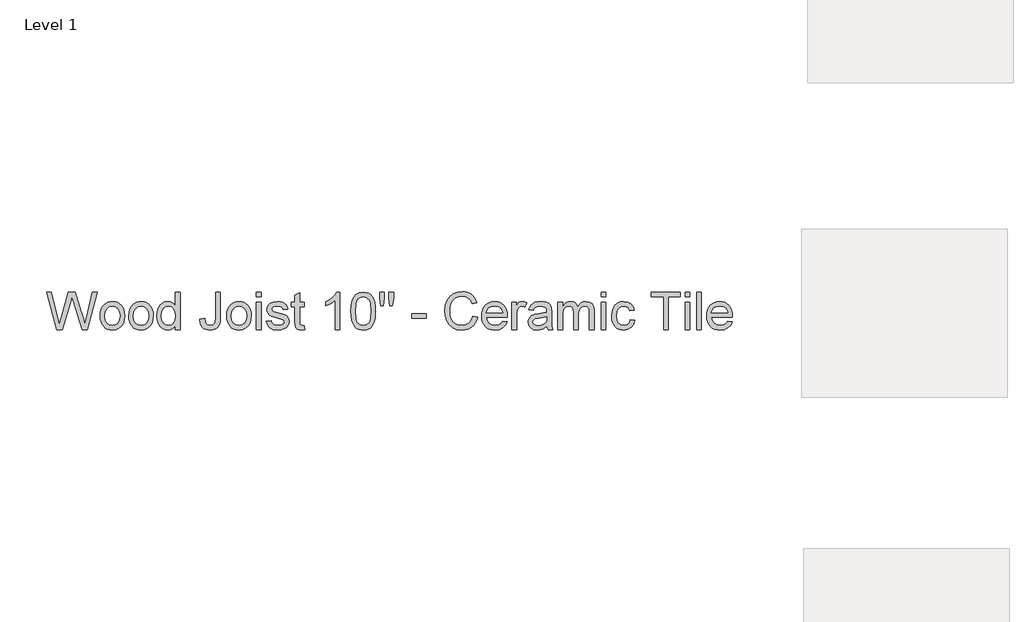
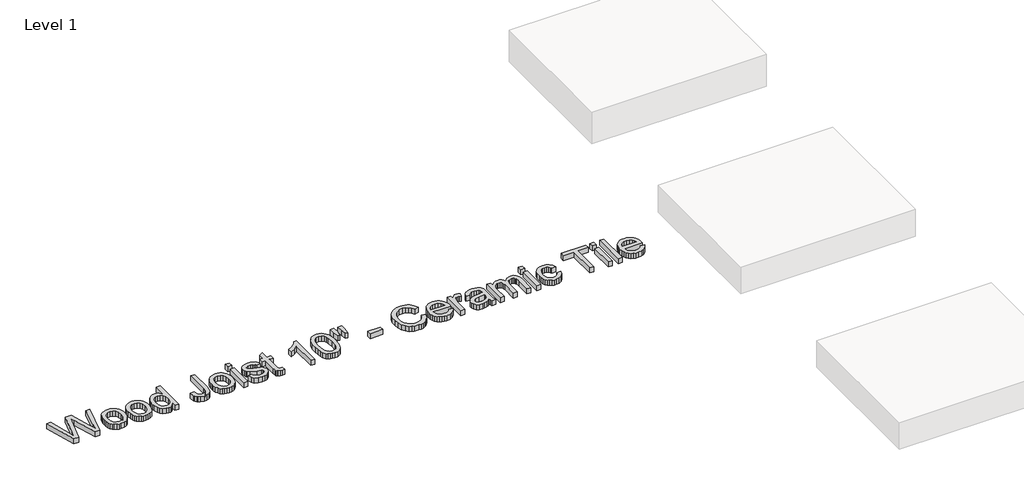
# One storey, part 15 of 42: 1 proxy.
"""IFC4 building model written with IfcOpenShell, lengths in millimetres."""

from ifc_helpers import new_model, si_unit, origin, origin_with_axes, place, context, project, spatial, polyline, outline, extrude, element, save

model = new_model("IFC4")

# Units and contexts
model_context = context("Model", 3, world=origin())
ifc_project = project(units=[si_unit("LENGTHUNIT", "METRE", prefix="MILLI")], contexts=[model_context])

# Site, building, storey
site = spatial("IfcSite", under=ifc_project)
building = spatial("IfcBuilding", under=site)
storey = spatial("IfcBuildingStorey", under=building, Name="Level 1", Elevation=0.0)

# Proxy
placement = place(None, origin())
element("IfcBuildingElementProxy", 1, Name="8\" Arial", ObjectType="8\" Arial", at=placement, inside=storey, context=model_context, shape_type="SweptSolid", body=[
    extrude(outline(polyline([(28459.9813839, -11347.8808193), (28376.9243908, -11043.3137252), (28416.1849927, -11043.3137252), (28464.3684588, -11243.4833095), (28479.2398989, -11305.2741433), (28495.1523399, -11250.6216008), (28555.5303868, -11043.3137252), (28612.1162166, -11043.3137252), (28655.986965, -11193.5896278), (28674.7807475, -11249.3575284), (28688.6297761, -11305.2741433), (28703.055073, -11245.2678823), (28751.6846823, -11043.3137252), (28790.9452843, -11043.3137252), (28707.8139339, -11347.8808193), (28667.1405451, -11347.8808193), (28594.121774, -11112.9120651), (28583.9348375, -11080.1205396), (28572.4838286, -11119.6042131), (28505.934134, -11347.8808193), (28459.9813839, -11347.8808193)])), origin_with_axes(), (0.0, 0.0, 1.0), 50.8),
    extrude(outline(polyline([(28814.7395885, -11236.0475894), (28816.7983535, -11207.0808124), (28822.9746485, -11182.1200296), (28833.2684734, -11161.165241), (28847.6798284, -11144.2164466), (28862.1887772, -11133.3835319), (28878.2034593, -11125.6457357), (28895.7238747, -11121.003058), (28914.7500234, -11119.4554987), (28935.753609, -11121.339989), (28954.7449027, -11126.99346), (28971.7239048, -11136.4159115), (28986.6906151, -11149.6073436), (28998.906109, -11166.1216132), (29007.6314617, -11185.5125769), (29012.8666734, -11207.7802349), (29014.611744, -11232.924587), (29011.5259201, -11271.3858491), (29002.2684486, -11300.6639968), (28987.1088743, -11322.5900764), (28966.3167421, -11338.9951338), (28941.6208568, -11349.2285435), (28914.7500234, -11352.6396801), (28893.4397144, -11350.7621608), (28874.2718223, -11345.1296029), (28857.246347, -11335.7420063), (28842.3632885, -11322.599371), (28830.2779198, -11305.9247688), (28821.6455135, -11285.9412711), (28816.4660697, -11262.648878), (28814.7395885, -11236.0475894)]), holes=[polyline([(28852.8104752, -11235.9732322), (28857.2161394, -11270.4285001), (28870.4331318, -11294.975671), (28890.323683, -11309.6705128), (28914.7500234, -11314.5687934), (28939.064828, -11309.6426288), (28958.9182006, -11294.8641352), (28972.1351931, -11269.9916516), (28976.5408572, -11234.783517), (28972.1073091, -11201.3320714), (28958.8066648, -11177.1195079), (28938.9254083, -11162.4246661), (28914.7500234, -11157.5263855), (28890.323683, -11162.4060768), (28870.4331318, -11177.0451507), (28857.2161394, -11201.5365537), (28852.8104752, -11235.9732322)])]), origin_with_axes(), (0.0, 0.0, 1.0), 50.8),
    extrude(outline(polyline([(29047.9237699, -11236.0475894), (29049.9825349, -11207.0808124), (29056.1588299, -11182.1200296), (29066.4526548, -11161.165241), (29080.8640098, -11144.2164466), (29095.3729586, -11133.3835319), (29111.3876407, -11125.6457357), (29128.9080561, -11121.003058), (29147.9342048, -11119.4554987), (29168.9377903, -11121.339989), (29187.9290841, -11126.99346), (29204.9080862, -11136.4159115), (29219.8747965, -11149.6073436), (29232.0902904, -11166.1216132), (29240.8156431, -11185.5125769), (29246.0508548, -11207.7802349), (29247.7959254, -11232.924587), (29244.7101015, -11271.3858491), (29235.45263, -11300.6639968), (29220.2930557, -11322.5900764), (29199.5009235, -11338.9951338), (29174.8050382, -11349.2285435), (29147.9342048, -11352.6396801), (29126.6238958, -11350.7621608), (29107.4560037, -11345.1296029), (29090.4305284, -11335.7420063), (29075.5474699, -11322.599371), (29063.4621012, -11305.9247688), (29054.8296949, -11285.9412711), (29049.6502511, -11262.648878), (29047.9237699, -11236.0475894)]), holes=[polyline([(29085.9946566, -11235.9732322), (29090.4003208, -11270.4285001), (29103.6173132, -11294.975671), (29123.5078644, -11309.6705128), (29147.9342048, -11314.5687934), (29172.2490094, -11309.6426288), (29192.102382, -11294.8641352), (29205.3193745, -11269.9916516), (29209.7250386, -11234.783517), (29205.2914905, -11201.3320714), (29191.9908462, -11177.1195079), (29172.1095897, -11162.4246661), (29147.9342048, -11157.5263855), (29123.5078644, -11162.4060768), (29103.6173132, -11177.0451507), (29090.4003208, -11201.5365537), (29085.9946566, -11235.9732322)])]), origin_with_axes(), (0.0, 0.0, 1.0), 50.8),
    extrude(outline(polyline([(29428.6326375, -11347.8808193), (29428.6326375, -11311.9662913), (29417.2420438, -11329.7608989), (29403.4441357, -11342.4713329), (29387.2389133, -11350.0975933), (29368.6263765, -11352.6396801), (29344.0141431, -11348.9589987), (29321.4839112, -11337.9169544), (29302.4112893, -11320.2850032), (29288.1718853, -11296.834601), (29279.3047892, -11268.5138022), (29276.3490904, -11236.270661), (29279.0724229, -11204.4271898), (29287.2424203, -11175.6695425), (29300.8497881, -11151.6335773), (29319.8852314, -11133.9551529), (29342.9080797, -11123.0804123), (29368.4776621, -11119.4554987), (29387.1041409, -11122.0487061), (29403.5742608, -11129.8283282), (29417.5348253, -11141.7533643), (29428.6326375, -11156.7828135), (29428.6326375, -11043.3137252), (29466.7035242, -11043.3137252), (29466.7035242, -11347.8808193), (29428.6326375, -11347.8808193)]), holes=[polyline([(29314.4199772, -11236.1219466), (29318.7141055, -11270.5586252), (29331.5964905, -11295.0500282), (29350.3159158, -11309.6891021), (29372.1211649, -11314.5687934), (29393.9171194, -11309.9121737), (29412.1625175, -11295.9423146), (29424.5151075, -11272.3989659), (29428.6326375, -11239.0218775), (29424.4407503, -11202.5310812), (29411.8650887, -11177.2310437), (29393.1549581, -11162.45255), (29370.5596637, -11157.5263855), (29348.531343, -11162.2573624), (29330.4811325, -11176.4502931), (29318.435266, -11200.8301603), (29314.4199772, -11236.1219466)])]), origin_with_axes(), (0.0, 0.0, 1.0), 50.8),
    extrude(outline(polyline([(29628.5047929, -11262.3700385), (29666.5756797, -11257.4624632), (29670.5352006, -11285.1419312), (29679.5881898, -11302.4485697), (29693.4186292, -11311.5387374), (29711.7105005, -11314.5687934), (29725.7733061, -11312.8492831), (29737.7726994, -11307.6907523), (29747.0301709, -11299.5672281), (29752.8672111, -11288.9527377), (29756.9940358, -11251.2164584), (29756.9940358, -11043.3137252), (29795.0649225, -11043.3137252), (29795.0649225, -11250.5472436), (29792.7691439, -11284.4448324), (29785.8818082, -11309.6983967), (29774.0032454, -11328.1482772), (29756.7337855, -11341.6348144), (29735.0493669, -11349.8884637), (29709.9259277, -11352.6396801), (29674.7363825, -11346.9606489), (29660.6410456, -11339.8618599), (29648.8786659, -11329.9235553), (29639.658373, -11317.1829137), (29633.1892966, -11301.6771137), (29628.5047929, -11262.3700385)])), origin_with_axes(), (0.0, 0.0, 1.0), 50.8),
    extrude(outline(polyline([(29847.4123918, -11236.0475894), (29849.4711568, -11207.0808124), (29855.6474518, -11182.1200296), (29865.9412768, -11161.165241), (29880.3526317, -11144.2164466), (29894.8615805, -11133.3835319), (29910.8762626, -11125.6457357), (29928.396678, -11121.003058), (29947.4228267, -11119.4554987), (29968.4264123, -11121.339989), (29987.4177061, -11126.99346), (30004.3967081, -11136.4159115), (30019.3634184, -11149.6073436), (30031.5789123, -11166.1216132), (30040.3042651, -11185.5125769), (30045.5394767, -11207.7802349), (30047.2845473, -11232.924587), (30044.1987235, -11271.3858491), (30034.941252, -11300.6639968), (30019.7816777, -11322.5900764), (29998.9895454, -11338.9951338), (29974.2936601, -11349.2285435), (29947.4228267, -11352.6396801), (29926.1125178, -11350.7621608), (29906.9446256, -11345.1296029), (29889.9191503, -11335.7420063), (29875.0360919, -11322.599371), (29862.9507231, -11305.9247688), (29854.3183168, -11285.9412711), (29849.1388731, -11262.648878), (29847.4123918, -11236.0475894)]), holes=[polyline([(29885.4832786, -11235.9732322), (29889.8889427, -11270.4285001), (29903.1059351, -11294.975671), (29922.9964863, -11309.6705128), (29947.4228267, -11314.5687934), (29971.7376314, -11309.6426288), (29991.591004, -11294.8641352), (30004.8079964, -11269.9916516), (30009.2136605, -11234.783517), (30004.7801124, -11201.3320714), (29991.4794682, -11177.1195079), (29971.5982116, -11162.4246661), (29947.4228267, -11157.5263855), (29922.9964863, -11162.4060768), (29903.1059351, -11177.0451507), (29889.8889427, -11201.5365537), (29885.4832786, -11235.9732322)])]), origin_with_axes(), (0.0, 0.0, 1.0), 50.8),
    extrude(outline(polyline([(30090.1142949, -11347.8808193), (30090.1142949, -11124.2143596), (30128.1851816, -11124.2143596), (30128.1851816, -11347.8808193), (30090.1142949, -11347.8808193)])), origin_with_axes(), (0.0, 0.0, 1.0), 50.8),
    extrude(outline(polyline([(30090.1142949, -11081.384612), (30090.1142949, -11043.3137252), (30128.1851816, -11043.3137252), (30128.1851816, -11081.384612), (30090.1142949, -11081.384612)])), origin_with_axes(), (0.0, 0.0, 1.0), 50.8),
    extrude(outline(polyline([(30171.0149292, -11281.2567675), (30209.085816, -11276.4979066), (30215.09016, -11292.7821336), (30226.7084726, -11304.7536429), (30244.015111, -11312.1150057), (30267.0844326, -11314.5687934), (30289.8749146, -11312.3194881), (30305.8988913, -11305.5715721), (30315.3794344, -11295.7936002), (30318.5396154, -11284.4541271), (30315.3608451, -11274.7505124), (30305.8245341, -11267.3519709), (30266.6382893, -11256.4958196), (30209.3088876, -11237.8693409), (30194.7999388, -11228.5096282), (30184.2876896, -11216.1198596), (30177.902265, -11201.4900804), (30175.7737901, -11185.4103358), (30177.4840057, -11170.6597261), (30182.6146526, -11157.0430637), (30190.7009981, -11145.0994383), (30201.2783099, -11135.3679397), (30225.4815788, -11124.1028238), (30258.2359257, -11119.4554987), (30283.0154628, -11121.3237234), (30304.5604617, -11126.9283974), (30321.8856895, -11135.7211364), (30334.0059132, -11147.153556), (30342.0364909, -11162.0714694), (30347.0927805, -11181.3206897), (30309.0218937, -11186.0795506), (30304.2165597, -11174.0987466), (30294.7081326, -11165.0736414), (30280.4036661, -11159.4131995), (30261.2102137, -11157.5263855), (30239.3491967, -11159.3295476), (30224.7751854, -11164.739034), (30216.577304, -11172.54654), (30213.8446769, -11181.5437613), (30218.3804661, -11192.6229842), (30232.5826914, -11201.0253479), (30265.3742169, -11209.1302828), (30321.2536533, -11227.0503681), (30336.0135576, -11235.6200355), (30347.2043163, -11247.3498839), (30354.2589557, -11262.277092), (30356.6105022, -11280.4388383), (30353.8499911, -11299.2140314), (30345.5684579, -11316.8738666), (30332.0819206, -11332.0334409), (30313.7063974, -11343.3078514), (30291.510773, -11350.306723), (30266.5639321, -11352.6396801), (30228.1770273, -11348.1410695), (30200.1629519, -11334.6452376), (30181.4621159, -11312.3008988), (30171.0149292, -11281.2567675)])), origin_with_axes(), (0.0, 0.0, 1.0), 50.8),
    extrude(outline(polyline([(30480.3408842, -11316.1302946), (30485.099745, -11348.9961773), (30456.6209371, -11352.6396801), (30438.3476551, -11351.0595896), (30424.721698, -11346.3193181), (30415.0924405, -11339.0137231), (30408.8092571, -11329.7376623), (30405.3516473, -11313.8066321), (30404.1991106, -11286.5361287), (30404.1991106, -11162.2852463), (30375.6459456, -11162.2852463), (30375.6459456, -11124.2143596), (30404.1991106, -11124.2143596), (30404.1991106, -11069.8592459), (30442.2699974, -11047.4777285), (30442.2699974, -11124.2143596), (30480.3408842, -11124.2143596), (30480.3408842, -11162.2852463), (30442.2699974, -11162.2852463), (30442.2699974, -11285.4207707), (30444.2776418, -11305.0510717), (30450.7838969, -11312.0034699), (30463.7592284, -11314.5687934), (30480.3408842, -11316.1302946)])), origin_with_axes(), (0.0, 0.0, 1.0), 50.8),
    extrude(outline(polyline([(30770.6313957, -11347.8808193), (30732.5605089, -11347.8808193), (30732.5605089, -11110.5326347), (30696.4972666, -11136.2230475), (30656.4187354, -11155.4443839), (30656.4187354, -11119.4554987), (30686.3196248, -11103.1898611), (30712.2238145, -11083.8383996), (30732.6441608, -11063.2600443), (30746.0935195, -11043.3137252), (30770.6313957, -11043.3137252), (30770.6313957, -11347.8808193)])), origin_with_axes(), (0.0, 0.0, 1.0), 50.8),
    extrude(outline(polyline([(30861.0497517, -11198.0510599), (30863.8474414, -11149.3006202), (30872.2405105, -11110.4210989), (30886.145307, -11080.8176383), (30905.4781792, -11059.895381), (30930.3785468, -11047.4591392), (30960.9858295, -11043.3137252), (30984.4455263, -11045.7675128), (31005.4514355, -11053.1288757), (31023.0183242, -11065.1096797), (31036.1609594, -11081.4217906), (31046.0876457, -11101.9257887), (31054.0066876, -11126.4822542), (31059.1931023, -11157.6658052), (31060.9219072, -11198.0510599), (31058.1521015, -11246.5226601), (31049.8426843, -11285.3092349), (31036.0215396, -11314.9405794), (31016.7165514, -11335.9464886), (30991.7604159, -11348.4663822), (30960.9858295, -11352.6396801), (30940.0170989, -11350.8272234), (30921.4277987, -11345.3898531), (30905.217929, -11336.3275692), (30891.3874896, -11323.6403719), (30878.1147293, -11300.7058228), (30868.6341862, -11272.1294211), (30862.9458604, -11237.9111668), (30861.0497517, -11198.0510599)]), holes=[polyline([(30899.1206385, -11197.9767027), (30903.5820705, -11257.8621332), (30909.1588606, -11278.3452183), (30916.9663667, -11292.5218834), (30936.8940965, -11309.0570659), (30960.9858295, -11314.5687934), (30985.0775625, -11309.0384766), (31005.0052923, -11292.4475262), (31012.8127984, -11278.2476245), (31018.3895884, -11257.7691867), (31022.8510205, -11197.9767027), (31018.5383028, -11139.4389964), (31013.1474058, -11119.0232975), (31005.6001499, -11104.5097014), (30985.7095987, -11087.1658843), (30960.5396863, -11081.384612), (30936.7082035, -11086.4780802), (30917.5612243, -11101.758485), (30909.493468, -11117.5593901), (30903.7307849, -11138.8627281), (30899.1206385, -11197.9767027)])]), origin_with_axes(), (0.0, 0.0, 1.0), 50.8),
    extrude(outline(polyline([(31103.5285832, -11152.7675246), (31094.2339331, -11093.9509789), (31094.2339331, -11043.3137252), (31132.3048199, -11043.3137252), (31132.3048199, -11093.9509789), (31123.9768134, -11152.7675246), (31103.5285832, -11152.7675246)])), origin_with_axes(), (0.0, 0.0, 1.0), 50.8),
    extrude(outline(polyline([(31179.4472851, -11152.7675246), (31170.3757067, -11093.9509789), (31170.3757067, -11043.3137252), (31208.4465934, -11043.3137252), (31208.4465934, -11093.9509789), (31199.5237293, -11152.7675246), (31179.4472851, -11152.7675246)])), origin_with_axes(), (0.0, 0.0, 1.0), 50.8),
    extrude(outline(polyline([(31355.9712796, -11257.4624632), (31355.9712796, -11219.3915765), (31474.9428007, -11219.3915765), (31474.9428007, -11257.4624632), (31355.9712796, -11257.4624632)])), origin_with_axes(), (0.0, 0.0, 1.0), 50.8),
    extrude(outline(polyline([(31855.6516683, -11239.6167351), (31893.7225551, -11249.4318856), (31886.1892412, -11273.107683), (31876.1556664, -11293.7952504), (31863.6218308, -11311.4945879), (31848.5877342, -11326.2056953), (31831.3926316, -11337.7705637), (31812.3757775, -11346.0311839), (31791.537172, -11350.9875561), (31768.8768151, -11352.6396801), (31724.7179325, -11347.6391584), (31706.0473042, -11341.3885062), (31689.6492178, -11332.6375931), (31662.7690897, -11308.1554848), (31643.1759673, -11274.7133338), (31631.2137527, -11235.3969639), (31627.2263478, -11193.292199), (31631.7342531, -11148.8823609), (31645.2579689, -11110.5326347), (31667.091102, -11079.4606194), (31696.5272588, -11056.8839143), (31731.4379645, -11043.1371269), (31769.6947443, -11038.5548644), (31791.4697858, -11040.0373611), (31811.4370178, -11044.4848511), (31829.5964405, -11051.8973346), (31845.9480536, -11062.2748114), (31860.2223125, -11075.3430894), (31872.1496722, -11090.8279765), (31888.9636942, -11129.0475776), (31850.8928075, -11138.1191561), (31837.6944043, -11110.3560363), (31819.6627832, -11091.3112983), (31796.5748724, -11080.2971379), (31768.2076003, -11076.6257511), (31735.5090213, -11080.6968079), (31708.6474825, -11092.9099781), (31688.2643149, -11111.9826001), (31675.0008492, -11136.6320121), (31667.7231382, -11164.4973731), (31665.2972345, -11193.2178418), (31668.1692814, -11228.3887978), (31676.785422, -11258.8008928), (31691.4709692, -11283.2922958), (31712.5512356, -11300.7011754), (31737.8233892, -11311.1018889), (31765.0845979, -11314.5687934), (31796.8630065, -11309.8471111), (31823.3434646, -11295.6820644), (31843.3362569, -11272.2223676), (31855.6516683, -11239.6167351)])), origin_with_axes(), (0.0, 0.0, 1.0), 50.8),
    extrude(outline(polyline([(32097.9074282, -11281.2567675), (32135.2347429, -11286.0156283), (32121.7853843, -11314.1412395), (32100.3240372, -11335.165738), (32071.3340236, -11348.2711946), (32035.2986652, -11352.6396801), (32011.676312, -11350.7551898), (31990.6285769, -11345.1017189), (31972.1554598, -11335.6792674), (31956.2569609, -11322.4878352), (31943.4721697, -11305.8945612), (31934.340176, -11286.2665839), (31928.8609797, -11263.6039033), (31927.034581, -11237.9065195), (31928.879569, -11211.3377622), (31934.4145332, -11187.9198913), (31943.6394734, -11167.6529068), (31956.5543897, -11150.5368086), (31972.4110627, -11136.9387356), (31990.4612732, -11127.2258262), (32010.7050211, -11121.3980806), (32033.1423064, -11119.4554987), (32054.8569327, -11121.3934333), (32074.4942046, -11127.2072369), (32092.0541223, -11136.8969096), (32107.5366857, -11150.4624514), (32120.1750861, -11167.541371), (32129.202515, -11187.7711769), (32134.6189724, -11211.1518692), (32136.4244582, -11237.6834478), (32136.2013866, -11247.9447415), (31965.1054677, -11247.9447415), (31971.6953747, -11276.4421387), (31987.0036634, -11297.39228), (32009.0970466, -11310.274665), (32036.0422372, -11314.5687934), (32056.3045744, -11312.5797383), (32073.369552, -11306.6125729), (32087.2371699, -11296.2955113), (32097.9074282, -11281.2567675)]), holes=[polyline([(31965.1054677, -11209.8738548), (32098.3535714, -11209.8738548), (32093.2043353, -11189.760232), (32083.1103453, -11175.3721137), (32060.9147208, -11161.9878175), (32032.993592, -11157.5263855), (32007.3310631, -11161.0862365), (31986.1113769, -11171.7657894), (31971.3607673, -11188.4125077), (31965.1054677, -11209.8738548)])]), origin_with_axes(), (0.0, 0.0, 1.0), 50.8),
    extrude(outline(polyline([(32174.4953449, -11347.8808193), (32174.4953449, -11124.2143596), (32207.8073708, -11124.2143596), (32207.8073708, -11157.3033139), (32220.1134875, -11138.1191561), (32231.4529607, -11126.8168616), (32242.8296124, -11121.2958395), (32255.2472649, -11119.4554987), (32274.2083511, -11122.3926082), (32293.466866, -11131.2039364), (32280.7517847, -11165.3338916), (32267.3674886, -11159.478262), (32253.9831925, -11157.5263855), (32242.6158354, -11159.4039048), (32232.4567829, -11165.0364628), (32224.2496068, -11173.9965054), (32218.7378793, -11185.856479), (32214.1091436, -11207.1226384), (32212.5662317, -11230.322085), (32212.5662317, -11347.8808193), (32174.4953449, -11347.8808193)])), origin_with_axes(), (0.0, 0.0, 1.0), 50.8),
    extrude(outline(polyline([(32460.0269956, -11319.3276542), (32441.8373654, -11334.9240771), (32423.1086455, -11345.1296029), (32403.4132819, -11350.7621608), (32382.3237209, -11352.6396801), (32350.5081336, -11348.1224802), (32327.0391422, -11334.5708804), (32312.567372, -11313.9925251), (32307.7434486, -11288.3950587), (32309.5652, -11272.6127429), (32315.0304542, -11258.2803924), (32323.4607019, -11246.0114543), (32334.1774334, -11236.4193754), (32360.8344899, -11223.9273657), (32393.7747298, -11218.2018613), (32432.7007243, -11212.178928), (32459.803924, -11205.1149939), (32460.0269956, -11196.6382731), (32457.4059043, -11179.6476527), (32449.5426303, -11168.5312512), (32431.9571523, -11160.2776019), (32407.4564547, -11157.5263855), (32384.7775085, -11159.3574316), (32368.9394247, -11164.8505698), (32358.1390413, -11175.0096223), (32350.5731962, -11190.8384114), (32312.5023094, -11186.0795506), (32319.1108056, -11165.2595344), (32328.9724294, -11148.9009502), (32343.007351, -11136.3903512), (32362.1357409, -11127.1142904), (32385.5303752, -11121.3701967), (32412.36403, -11119.4554987), (32438.1009161, -11121.1471251), (32458.502673, -11126.222004), (32473.8853189, -11133.8529117), (32484.5648718, -11143.2126244), (32491.6473952, -11154.7844637), (32496.2389523, -11169.0517516), (32498.0978824, -11202.3637775), (32498.0978824, -11249.7293144), (32500.0311696, -11315.8700444), (32507.6156041, -11347.8808193), (32469.5447173, -11347.8808193), (32463.4474268, -11334.6452376), (32460.0269956, -11319.3276542)]), holes=[polyline([(32460.0269956, -11243.1858807), (32398.6079478, -11254.8599612), (32365.8536009, -11261.0316089), (32351.0193394, -11271.069831), (32345.8143353, -11285.7181995), (32348.6492036, -11297.0390833), (32357.1538084, -11306.3151441), (32371.1422568, -11312.5053811), (32390.4286558, -11314.5687934), (32410.8768859, -11312.2916041), (32428.9456857, -11305.4600363), (32443.5940543, -11295.3939302), (32453.7809907, -11283.4131263), (32458.2981907, -11271.069831), (32459.803924, -11253.9676748), (32460.0269956, -11243.1858807)])]), origin_with_axes(), (0.0, 0.0, 1.0), 50.8),
    extrude(outline(polyline([(32550.4453517, -11347.8808193), (32550.4453517, -11124.2143596), (32588.5162384, -11124.2143596), (32588.5162384, -11161.0211739), (32599.9672473, -11144.1142054), (32614.6899731, -11130.869329), (32632.1825045, -11122.3089563), (32651.9429306, -11119.4554987), (32673.1161435, -11122.3647242), (32690.0881746, -11131.0924006), (32702.7660773, -11145.0622597), (32711.0569052, -11163.6980332), (32724.9338178, -11144.3419243), (32740.7626069, -11130.5161323), (32758.5432725, -11122.2206571), (32778.2758146, -11119.4554987), (32806.8940422, -11124.0563505), (32828.0579605, -11137.8589059), (32841.1355331, -11161.2349509), (32845.494724, -11194.5562714), (32845.494724, -11347.8808193), (32807.4238373, -11347.8808193), (32807.4238373, -11210.9148556), (32803.8918702, -11179.1271523), (32798.9285271, -11170.3622973), (32791.1024317, -11163.4749615), (32781.0363257, -11159.0135295), (32769.3529505, -11157.5263855), (32748.728122, -11161.337192), (32731.9141, -11172.7696116), (32720.7326359, -11192.6043949), (32717.0054812, -11221.6222925), (32717.0054812, -11347.8808193), (32678.9345945, -11347.8808193), (32678.9345945, -11206.6764952), (32676.7317624, -11185.1500856), (32670.1232662, -11169.7953236), (32658.4956589, -11160.59362), (32641.2354937, -11157.5263855), (32626.5685359, -11159.5712085), (32613.0541146, -11165.7056776), (32601.9005345, -11175.7810783), (32594.3161001, -11189.6486962), (32589.9662038, -11208.8886219), (32588.5162384, -11235.0809458), (32588.5162384, -11347.8808193), (32550.4453517, -11347.8808193)])), origin_with_axes(), (0.0, 0.0, 1.0), 50.8),
    extrude(outline(polyline([(32902.6010542, -11081.384612), (32902.6010542, -11043.3137252), (32940.6719409, -11043.3137252), (32940.6719409, -11081.384612), (32902.6010542, -11081.384612)])), origin_with_axes(), (0.0, 0.0, 1.0), 50.8),
    extrude(outline(polyline([(32902.6010542, -11347.8808193), (32902.6010542, -11124.2143596), (32940.6719409, -11124.2143596), (32940.6719409, -11347.8808193), (32902.6010542, -11347.8808193)])), origin_with_axes(), (0.0, 0.0, 1.0), 50.8),
    extrude(outline(polyline([(33140.5440964, -11266.9801849), (33178.6149832, -11271.7390458), (33168.0004928, -11305.599456), (33148.0541737, -11331.1876277), (33120.6535452, -11347.276667), (33087.6761267, -11352.6396801), (33066.3239918, -11350.7691318), (33047.1793363, -11345.1574868), (33030.2421602, -11335.8047452), (33015.5124634, -11322.7109068), (33003.589751, -11306.1222801), (32995.0735279, -11286.2851732), (32989.963794, -11263.199586), (32988.2605494, -11236.8655186), (32991.1697749, -11202.9865191), (32999.8974513, -11173.6247194), (33014.5829984, -11149.9140671), (33035.365836, -11132.9885093), (33060.229025, -11122.8387514), (33087.1556263, -11119.4554987), (33119.3244103, -11124.1028238), (33145.0427071, -11138.0447989), (33163.4925875, -11160.5378521), (33173.8561223, -11190.8384114), (33135.7852356, -11195.5972723), (33128.8793106, -11178.9877325), (33118.1254004, -11167.0812858), (33104.1183627, -11159.9151106), (33087.4530551, -11157.5263855), (33062.8501163, -11162.2294784), (33043.3220565, -11176.3387573), (33030.5790912, -11200.6163833), (33026.3314361, -11235.8245178), (33030.4861447, -11271.5066795), (33042.9502705, -11295.8679574), (33062.1251336, -11309.8935844), (33086.4120543, -11314.5687934), (33106.1260071, -11311.6502732), (33122.2894036, -11302.8947129), (33134.047136, -11288.0790406), (33140.5440964, -11266.9801849)])), origin_with_axes(), (0.0, 0.0, 1.0), 50.8),
    extrude(outline(polyline([(33411.7991646, -11347.8808193), (33411.7991646, -11081.384612), (33311.8630868, -11081.384612), (33311.8630868, -11043.3137252), (33549.8061291, -11043.3137252), (33549.8061291, -11081.384612), (33449.8700513, -11081.384612), (33449.8700513, -11347.8808193), (33411.7991646, -11347.8808193)])), origin_with_axes(), (0.0, 0.0, 1.0), 50.8),
    extrude(outline(polyline([(33587.8770158, -11081.384612), (33587.8770158, -11043.3137252), (33625.9479026, -11043.3137252), (33625.9479026, -11081.384612), (33587.8770158, -11081.384612)])), origin_with_axes(), (0.0, 0.0, 1.0), 50.8),
    extrude(outline(polyline([(33587.8770158, -11347.8808193), (33587.8770158, -11124.2143596), (33625.9479026, -11124.2143596), (33625.9479026, -11347.8808193), (33587.8770158, -11347.8808193)])), origin_with_axes(), (0.0, 0.0, 1.0), 50.8),
    extrude(outline(polyline([(33683.0542327, -11347.8808193), (33683.0542327, -11043.3137252), (33721.1251195, -11043.3137252), (33721.1251195, -11347.8808193), (33683.0542327, -11347.8808193)])), origin_with_axes(), (0.0, 0.0, 1.0), 50.8),
    extrude(outline(polyline([(33934.8277143, -11281.2567675), (33972.155029, -11286.0156283), (33958.7056704, -11314.1412395), (33937.2443233, -11335.165738), (33908.2543097, -11348.2711946), (33872.2189513, -11352.6396801), (33848.5965981, -11350.7551898), (33827.548863, -11345.1017189), (33809.0757459, -11335.6792674), (33793.177247, -11322.4878352), (33780.3924558, -11305.8945612), (33771.2604621, -11286.2665839), (33765.7812658, -11263.6039033), (33763.9548671, -11237.9065195), (33765.7998551, -11211.3377622), (33771.3348193, -11187.9198913), (33780.5597595, -11167.6529068), (33793.4746758, -11150.5368086), (33809.3313488, -11136.9387356), (33827.3815593, -11127.2258262), (33847.6253072, -11121.3980806), (33870.0625925, -11119.4554987), (33891.7772188, -11121.3934333), (33911.4144907, -11127.2072369), (33928.9744084, -11136.8969096), (33944.4569718, -11150.4624514), (33957.0953722, -11167.541371), (33966.1228011, -11187.7711769), (33971.5392585, -11211.1518692), (33973.3447443, -11237.6834478), (33973.1216727, -11247.9447415), (33802.0257538, -11247.9447415), (33808.6156608, -11276.4421387), (33823.9239495, -11297.39228), (33846.0173327, -11310.274665), (33872.9625233, -11314.5687934), (33893.2248605, -11312.5797383), (33910.2898381, -11306.6125729), (33924.157456, -11296.2955113), (33934.8277143, -11281.2567675)]), holes=[polyline([(33802.0257538, -11209.8738548), (33935.2738575, -11209.8738548), (33930.1246214, -11189.760232), (33920.0306314, -11175.3721137), (33897.8350069, -11161.9878175), (33869.9138781, -11157.5263855), (33844.2513492, -11161.0862365), (33823.031663, -11171.7657894), (33808.2810534, -11188.4125077), (33802.0257538, -11209.8738548)])]), origin_with_axes(), (0.0, 0.0, 1.0), 50.8),
])

save(model, "model.ifc")

# Revit data of these elements
# Element 1 (IfcBuildingElementProxy, "8\" Arial")
#   Phase Created = New Construction
